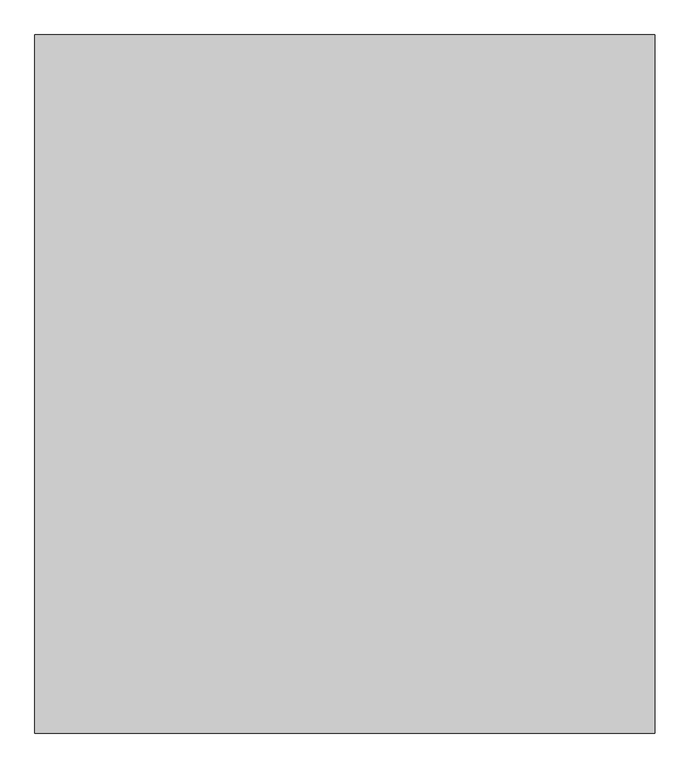
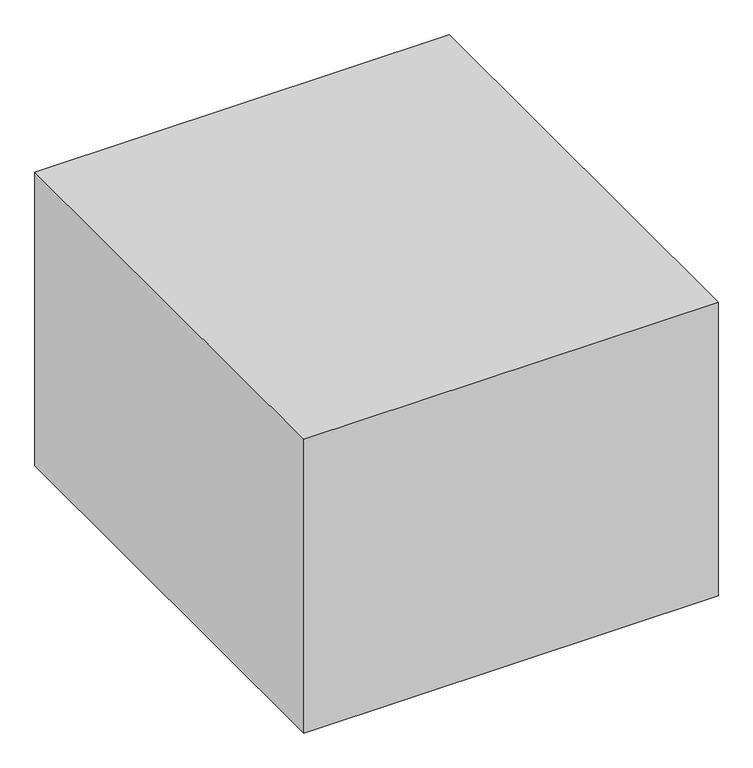
"""IFC4 building model written with IfcOpenShell, lengths in millimetres: proxy geometry, Space Planning Box_hec : Space Planning Box_hec."""

import ifcopenshell
import ifcopenshell.guid

model = None  # the IFC model being written
_history = None  # IfcOwnerHistory: only IFC2X3 demands one
_inside = {}  # id of a spatial element -> (the spatial element, [elements in it])
_under = {}  # id of a project, library or spatial element -> (it, [spatial elements below it])
_declared = {}  # id of a project -> (the project, [libraries it declares])
_typed = {}  # id of a type object -> (the type object, [elements of that type])
_made_of = {}  # id of a material, layer set ... -> (it, [elements and type objects made of it])


def new_model(schema):
    """Start an empty IFC model of exactly this schema.

    Asked for "IFC4X3", IfcOpenShell would pick the latest addendum, in which some entities
    have other attributes; the version numbers below select the first issue.
    IFC2X3 requires an IfcOwnerHistory on every rooted entity: one is made here for all.
    """
    global model, _history
    if schema == "IFC4X3":
        model = ifcopenshell.file(schema_version=(4, 3, 0, 0))
    else:
        model = ifcopenshell.file(schema=schema)
    _inside.clear()
    _under.clear()
    _declared.clear()
    _typed.clear()
    _made_of.clear()
    _history = None
    if model.schema == "IFC2X3":
        org = make("IfcOrganization", Name="unknown")
        user = make(
            "IfcPersonAndOrganization",
            ThePerson=make("IfcPerson", FamilyName="unknown"),
            TheOrganization=org,
        )
        app = make(
            "IfcApplication",
            ApplicationDeveloper=org,
            Version="unknown",
            ApplicationFullName="unknown",
            ApplicationIdentifier="unknown",
        )
        _history = make(
            "IfcOwnerHistory",
            OwningUser=user,
            OwningApplication=app,
            ChangeAction="ADDED",
            CreationDate=0,
        )
    return model


def make(cls, **values):
    """One entity of the class cls with the attributes given. An attribute that is None is left unset."""
    return model.create_entity(
        cls, **{name: value for name, value in values.items() if value is not None}
    )


def rooted(cls, **values):
    """An entity with a GlobalId (a new one), such as an element, a storey or a relation."""
    return make(cls, GlobalId=ifcopenshell.guid.new(), OwnerHistory=_history, **values)


def si_unit(unit_type, name, prefix=None):
    """IfcSIUnit, for example si_unit("LENGTHUNIT", "METRE", prefix="MILLI")."""
    return make("IfcSIUnit", UnitType=unit_type, Prefix=prefix, Name=name)


def assignment(units):
    """IfcUnitAssignment: the units of a project."""
    return None if units is None else make("IfcUnitAssignment", Units=units)


def point(xyz):
    """IfcCartesianPoint."""
    return None if xyz is None else make("IfcCartesianPoint", Coordinates=xyz)


def direction(xyz):
    """IfcDirection."""
    return None if xyz is None else make("IfcDirection", DirectionRatios=xyz)


def frame(location, z_axis=None, x_axis=None):
    """IfcAxis2Placement3D, a coordinate frame: its origin and axes. An axis left out is left unset."""
    return make(
        "IfcAxis2Placement3D",
        Location=point(location),
        Axis=direction(z_axis),
        RefDirection=direction(x_axis),
    )


def origin():
    """The frame at (0, 0, 0) with its axes left unset."""
    return frame((0.0, 0.0, 0.0))


def origin_with_axes():
    """The frame at (0, 0, 0) with the z axis (0, 0, 1) and the x axis (1, 0, 0) written out."""
    return frame((0.0, 0.0, 0.0), z_axis=(0.0, 0.0, 1.0), x_axis=(1.0, 0.0, 0.0))


def place(relative_to, where):
    """IfcLocalPlacement: puts the frame where relative to a parent placement (None: the world)."""
    return make(
        "IfcLocalPlacement", PlacementRelTo=relative_to, RelativePlacement=where
    )


def context(
    kind, dimensions, precision=None, world=None, true_north=None, identifier=None
):
    """IfcGeometricRepresentationContext, for example the 3D "Model" context."""
    return make(
        "IfcGeometricRepresentationContext",
        ContextIdentifier=identifier,
        ContextType=kind,
        CoordinateSpaceDimension=dimensions,
        Precision=precision,
        WorldCoordinateSystem=world,
        TrueNorth=true_north,
    )


def project(units=None, contexts=None):
    """IfcProject with its units and contexts."""
    return rooted(
        "IfcProject",
        Name="project",
        RepresentationContexts=contexts,
        UnitsInContext=assignment(units),
    )


def spatial(cls, under=None, at=None, **own):
    """A site, building, storey or space (cls), placed at a placement, below another one or the project."""
    s = rooted(cls, ObjectPlacement=at, **own)
    if under is not None:
        _under.setdefault(under.id(), (under, []))[1].append(s)
    return s


def polyline(points):
    """IfcPolyline through the points."""
    return make("IfcPolyline", Points=[point(p) for p in points])


def outline(outer, holes=None, kind="AREA"):
    """IfcArbitraryClosedProfileDef: a profile drawn as a closed curve; with holes, ...WithVoids."""
    if holes is None:
        return make("IfcArbitraryClosedProfileDef", ProfileType=kind, OuterCurve=outer)
    return make(
        "IfcArbitraryProfileDefWithVoids",
        ProfileType=kind,
        OuterCurve=outer,
        InnerCurves=holes,
    )


def extrude(swept, where, along, depth):
    """IfcExtrudedAreaSolid: the profile swept, set in the frame where, extruded along a direction by depth."""
    return make(
        "IfcExtrudedAreaSolid",
        SweptArea=swept,
        Position=where,
        ExtrudedDirection=direction(along),
        Depth=depth,
    )


def shape(context_of_items, identifier, shape_type, items):
    """IfcShapeRepresentation: the items that make up one representation, for example the "Body"."""
    return make(
        "IfcShapeRepresentation",
        ContextOfItems=context_of_items,
        RepresentationIdentifier=identifier,
        RepresentationType=shape_type,
        Items=items,
    )


def source(mapping_origin, context_of_items, identifier, shape_type, items):
    """IfcRepresentationMap: a shape defined once, which mapped items show again and again."""
    return make(
        "IfcRepresentationMap",
        MappingOrigin=mapping_origin,
        MappedRepresentation=shape(context_of_items, identifier, shape_type, items),
    )


def transform(
    local_origin,
    x_axis=None,
    y_axis=None,
    z_axis=None,
    scale=None,
    scale2=None,
    scale3=None,
    uniform=True,
):
    """IfcCartesianTransformationOperator3D, or its non-uniform kind. x_axis, y_axis, z_axis: its Axis1, 2, 3."""
    if uniform:
        return make(
            "IfcCartesianTransformationOperator3D",
            Axis1=direction(x_axis),
            Axis2=direction(y_axis),
            LocalOrigin=point(local_origin),
            Scale=scale,
            Axis3=direction(z_axis),
        )
    return make(
        "IfcCartesianTransformationOperator3DnonUniform",
        Axis1=direction(x_axis),
        Axis2=direction(y_axis),
        LocalOrigin=point(local_origin),
        Scale=scale,
        Axis3=direction(z_axis),
        Scale2=scale2,
        Scale3=scale3,
    )


def mapped(mapping_source, mapping_target):
    """IfcMappedItem: shows the shape of a source again, moved by a transform."""
    return make(
        "IfcMappedItem", MappingSource=mapping_source, MappingTarget=mapping_target
    )


def made_of(thing, what):
    """Note that an element or type object is made of a material, layer set ...; save() writes the relation."""
    if what is not None:
        _made_of.setdefault(what.id(), (what, []))[1].append(thing)
    return thing


def element(
    cls,
    number,
    at=None,
    inside=None,
    cuts=None,
    type_object=None,
    material=None,
    context=None,
    identifier="Body",
    shape_type=None,
    held_by="IfcProductDefinitionShape",
    body=None,
    shapes=None,
    **own,
):
    """One element of the class cls, such as IfcWall. Its Tag is "e" and its number.

    at: its placement. inside: the storey or other place that contains it. cuts: it is an
    opening in that element (IfcRelVoidsElement). A single representation is given by context,
    identifier, shape_type and body (its items); several are given by shapes. held_by: the class
    of the entity that holds the representations. save() writes the other relations.
    """
    e = rooted(cls, Tag="e%d" % number, ObjectPlacement=at, **own)
    if body is not None:
        shapes = [shape(context, identifier, shape_type, body)]
    if shapes is not None:
        e.Representation = make(held_by, Representations=shapes)
    if inside is not None:
        _inside.setdefault(inside.id(), (inside, []))[1].append(e)
    if cuts is not None:
        rooted(
            "IfcRelVoidsElement", RelatingBuildingElement=cuts, RelatedOpeningElement=e
        )
    if type_object is not None:
        _typed.setdefault(type_object.id(), (type_object, []))[1].append(e)
    return made_of(e, material)


def aggregate(whole, parts):
    """IfcRelAggregates: a whole, such as a stair, and the parts it consists of."""
    return rooted("IfcRelAggregates", RelatingObject=whole, RelatedObjects=parts)


def save(model, path):
    """Write the relations noted so far, then the file.

    IfcRelAggregates (storeys below a building ...), IfcRelContainedInSpatialStructure (elements
    in a storey), IfcRelDefinesByType, IfcRelAssociatesMaterial and IfcRelDeclares: one each for
    every whole, place, type object, material and project.
    """
    for whole, parts in _under.values():
        aggregate(whole, parts)
    for where, things in _inside.values():
        rooted(
            "IfcRelContainedInSpatialStructure",
            RelatedElements=things,
            RelatingStructure=where,
        )
    for kind, things in _typed.values():
        rooted("IfcRelDefinesByType", RelatedObjects=things, RelatingType=kind)
    for what, things in _made_of.values():
        rooted("IfcRelAssociatesMaterial", RelatedObjects=things, RelatingMaterial=what)
    for by, libraries in _declared.values():
        rooted("IfcRelDeclares", RelatingContext=by, RelatedDefinitions=libraries)
    model.write(path)


def generic_models_4d084078(model_context):
    return source(origin(), model_context, "Body", "SweptSolid", [
        extrude(outline(polyline([(4000.0, 4500.0), (4000.0, -4500.0), (-4000.0, -4500.0), (-4000.0, 4500.0), (4000.0, 4500.0)])), origin_with_axes(), (0.0, 0.0, 1.0), 6000.0),
    ])


if __name__ == "__main__":
    model = new_model("IFC4")
    model_context = context("Model", 3, world=origin())
    ifc_project = project(units=[si_unit("LENGTHUNIT", "METRE", prefix="MILLI")], contexts=[model_context])
    site = spatial("IfcSite", under=ifc_project)
    building = spatial("IfcBuilding", under=site)
    placement = place(None, origin())
    generic_models_shape = generic_models_4d084078(model_context)
    element("IfcBuildingElementProxy", 1, Name="Space Planning Box_hec : Space Planning Box_hec", ObjectType="Space Planning Box_hec : Space Planning Box_hec", at=placement, inside=building, context=model_context, shape_type="MappedRepresentation", body=[
        mapped(generic_models_shape, transform((0.0, 0.0, 0.0), x_axis=(1.0, 0.0, 0.0), y_axis=(0.0, 1.0, 0.0), z_axis=(0.0, 0.0, 1.0))),
    ])
    save(model, "model.ifc")

# Revit data of these elements
# Type "Space Planning Box_hec : Space Planning Box_hec"
#   Type Comments = "..."
#   Room Name [instance default] = "?"
#   Interior Finish [instance default] = ""
#   Exterior Finish [instance default] = ""
#   Department [instance default] = ""
#   Assembly Code = "..."
#   Width [instance default] = 1524 mm
#   Program Area [instance default] = 0.00 m²
#   Length [instance default] = 1524 mm
#   Height [instance default] = 1524 mm
#   Area [instance default] = 2.32258 m²
#   Fill Color [instance default] = Cyan
#   Default Elevation = 0
# Element 1 (IfcBuildingElementProxy, "Space Planning Box_hec : Space Planning Box_hec")
#   Room Name = "Fire Gas Room"
#   Interior Finish = "IF1"
#   Exterior Finish = "EF1"
#   Department = "SF"
#   Width = 8000 mm
#   Length = 9000 mm
#   Height = 6000 mm
#   Area = 72.00 m²
#   Materials on its faces: "Cyan"
# Materials
#   "Cyan": class "Generic", colour RGB 0 255 255, transparency 0.2, Cost = 0
